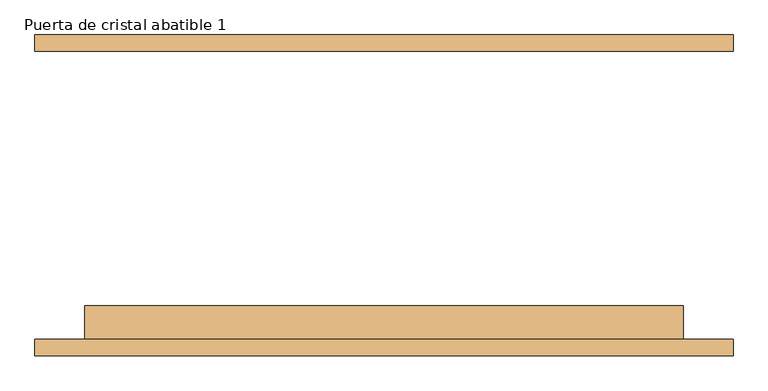
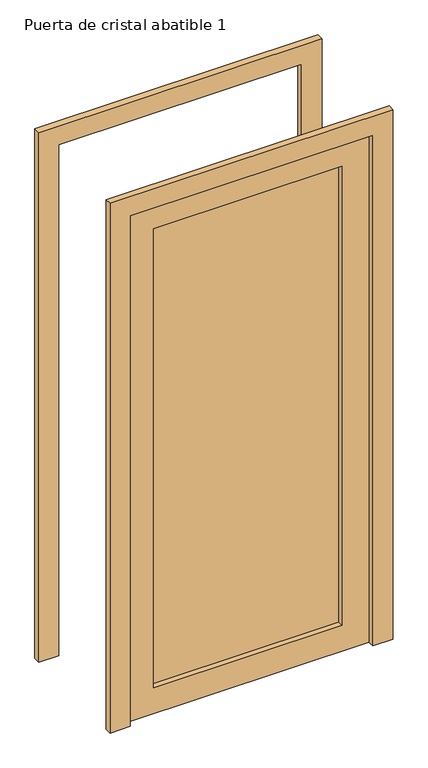
"""IFC4 building model written with IfcOpenShell, lengths in millimetres: door geometry, Puerta de cristal abatible 1 : PUERTA VIDRIO PABLO."""

from ifc_helpers import new_model, si_unit, frame, origin, place, context, project, spatial, polyline, outline, extrude, source, transform, mapped, element, save


def puerta_de_cristal_abatible_1_40d38811(model_context):
    return source(origin(), model_context, "Body", "SweptSolid", [
        extrude(outline(polyline([(2032.0, 457.5), (0.0, 457.5), (0.0, 533.5), (2108.0, 533.5), (2108.0, -533.5), (0.0, -533.5), (0.0, -457.5), (2032.0, -457.5), (2032.0, 457.5)])), frame((0.0, 220.0, 0.0), z_axis=(0.0, 1.0, 0.0), x_axis=(0.0, 0.0, 1.0)), (0.0, 0.0, 1.0), 25.0),
        extrude(outline(polyline([(2032.0, 457.5), (0.0, 457.5), (0.0, 533.5), (2108.0, 533.5), (2108.0, -533.5), (0.0, -533.5), (0.0, -457.5), (2032.0, -457.5), (2032.0, 457.5)])), frame((0.0, -245.0, 0.0), z_axis=(0.0, 1.0, 0.0), x_axis=(0.0, 0.0, 1.0)), (0.0, 0.0, 1.0), 25.0),
        extrude(outline(polyline([(355.5, -191.425), (355.5, -197.775), (-355.5, -197.775), (-355.5, -191.425), (355.5, -191.425)])), frame((0.0, 0.0, 102.0), z_axis=(0.0, 0.0, 1.0), x_axis=(1.0, 0.0, 0.0)), (0.0, 0.0, 1.0), 1828.0),
        extrude(outline(polyline([(2032.0, 457.5), (2032.0, -457.5), (0.0, -457.5), (0.0, 457.5), (2032.0, 457.5)]), holes=[polyline([(1930.0, -355.5), (1930.0, 355.5), (102.0, 355.5), (102.0, -355.5), (1930.0, -355.5)])]), frame((0.0, -220.0, 0.0), z_axis=(0.0, 1.0, 0.0), x_axis=(0.0, 0.0, 1.0)), (0.0, 0.0, 1.0), 51.0),
    ])


if __name__ == "__main__":
    model = new_model("IFC4")
    model_context = context("Model", 3, world=origin())
    ifc_project = project(units=[si_unit("LENGTHUNIT", "METRE", prefix="MILLI")], contexts=[model_context])
    site = spatial("IfcSite", under=ifc_project)
    building = spatial("IfcBuilding", under=site)
    placement = place(None, origin())
    puerta_de_cristal_abatible_1_shape = puerta_de_cristal_abatible_1_40d38811(model_context)
    element("IfcDoor", 1, ObjectType="Puerta de cristal abatible 1 : PUERTA VIDRIO PABLO", at=placement, inside=building, context=model_context, shape_type="MappedRepresentation", body=[
        mapped(puerta_de_cristal_abatible_1_shape, transform((0.0, 0.0, 0.0), x_axis=(1.0, 0.0, 0.0), y_axis=(0.0, 1.0, 0.0), z_axis=(0.0, 0.0, 1.0))),
    ])
    save(model, "model.ifc")

# Revit data of these elements
# Type "Puerta de cristal abatible 1 : PUERTA VIDRIO PABLO"
#   Description = "Puerta vidrio 1 hoja abatible"
#   Type Mark = "P2"
#   Construction Type Id = "SGL"
#   Analytic Construction = "Ventanas grandes con acristalamiento simple"
#   Visual Light Transmittance = 0.9
#   Thickness = 0.051 m
#   Solar Heat Gain Coefficient = 0.86
#   Heat Transfer Coefficient (U) = 5.5617 W/(m²·K)
#   Height = 2.032 m
#   Anchura de barandal - Base = 0.102 m
#   Anchura de barandal - Parte superior = 0.102 m
#   Anchura de montante - Bisagra = 0.102 m
#   Anchura de montante - Pasador = 0.102 m
#   Proyección cubrejuntas ext = 0.025 m
#   Proyección cubrejuntas int = 0.025 m
#   Anchura de cubrejuntas = 0.076 m
#   Width = 0.915 m
#   Define Thermal Properties by = 1
#   Material de puerta = Puerta - Panel
#   Material de estructura = Puerta - Marco
#   Function = (empty or 0)
#   Wall Closure = (empty or 0)
# Element 1 (IfcDoor, "Puerta de cristal abatible 1 : PUERTA VIDRIO PABLO")
#   Materials on its faces: "Puerta - Marco", "Puerta - Panel", "Vidrio"
# Materials
#   "Puerta - Panel": class "Madera", colour RGB 210 159 95, transparency 0
#   "Puerta - Marco": class "Madera", colour RGB 118 70 51, transparency 0
#   "Vidrio": class "Vidrio", colour RGB 0 128 192, transparency 0.75, Description = "Vidrio de cal sodada", Cost = 0
